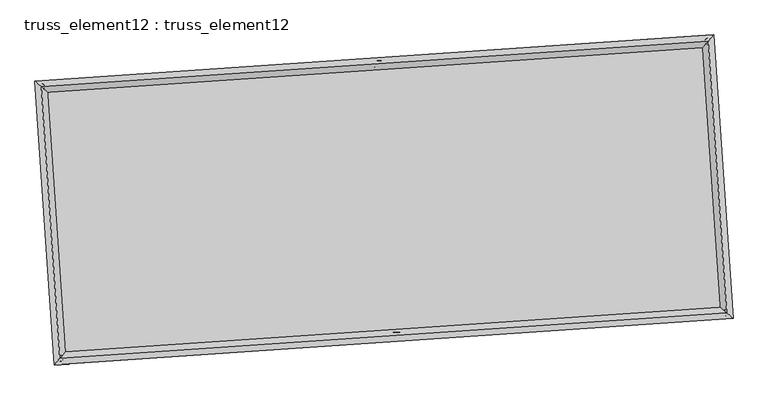
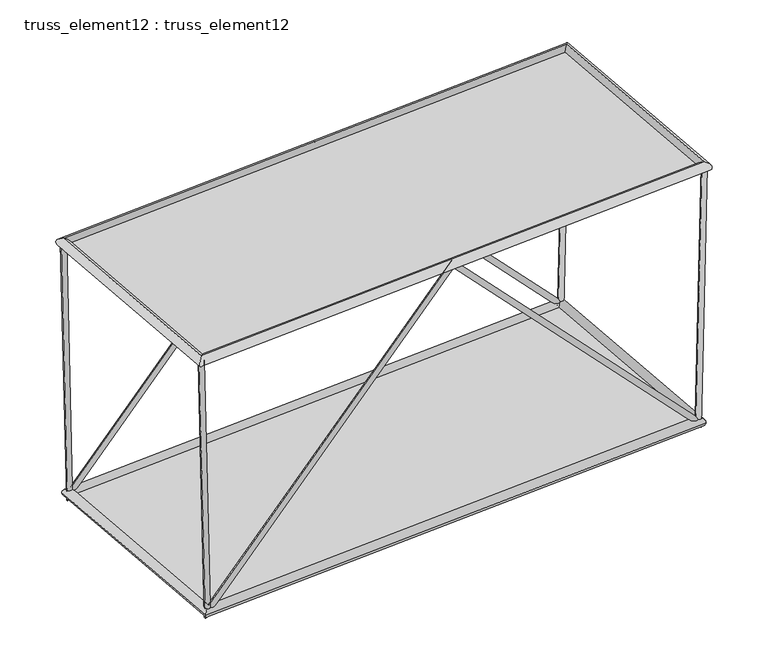
"""IFC4 building model written with IfcOpenShell, lengths in millimetres: plate geometry, truss_element12 : truss_element12."""

import ifcopenshell
import ifcopenshell.guid

model = None  # the IFC model being written
_history = None  # IfcOwnerHistory: only IFC2X3 demands one
_inside = {}  # id of a spatial element -> (the spatial element, [elements in it])
_under = {}  # id of a project, library or spatial element -> (it, [spatial elements below it])
_declared = {}  # id of a project -> (the project, [libraries it declares])
_typed = {}  # id of a type object -> (the type object, [elements of that type])
_made_of = {}  # id of a material, layer set ... -> (it, [elements and type objects made of it])


def new_model(schema):
    """Start an empty IFC model of exactly this schema.

    Asked for "IFC4X3", IfcOpenShell would pick the latest addendum, in which some entities
    have other attributes; the version numbers below select the first issue.
    IFC2X3 requires an IfcOwnerHistory on every rooted entity: one is made here for all.
    """
    global model, _history
    if schema == "IFC4X3":
        model = ifcopenshell.file(schema_version=(4, 3, 0, 0))
    else:
        model = ifcopenshell.file(schema=schema)
    _inside.clear()
    _under.clear()
    _declared.clear()
    _typed.clear()
    _made_of.clear()
    _history = None
    if model.schema == "IFC2X3":
        org = make("IfcOrganization", Name="unknown")
        user = make(
            "IfcPersonAndOrganization",
            ThePerson=make("IfcPerson", FamilyName="unknown"),
            TheOrganization=org,
        )
        app = make(
            "IfcApplication",
            ApplicationDeveloper=org,
            Version="unknown",
            ApplicationFullName="unknown",
            ApplicationIdentifier="unknown",
        )
        _history = make(
            "IfcOwnerHistory",
            OwningUser=user,
            OwningApplication=app,
            ChangeAction="ADDED",
            CreationDate=0,
        )
    return model


def make(cls, **values):
    """One entity of the class cls with the attributes given. An attribute that is None is left unset."""
    return model.create_entity(
        cls, **{name: value for name, value in values.items() if value is not None}
    )


def rooted(cls, **values):
    """An entity with a GlobalId (a new one), such as an element, a storey or a relation."""
    return make(cls, GlobalId=ifcopenshell.guid.new(), OwnerHistory=_history, **values)


def si_unit(unit_type, name, prefix=None):
    """IfcSIUnit, for example si_unit("LENGTHUNIT", "METRE", prefix="MILLI")."""
    return make("IfcSIUnit", UnitType=unit_type, Prefix=prefix, Name=name)


def assignment(units):
    """IfcUnitAssignment: the units of a project."""
    return None if units is None else make("IfcUnitAssignment", Units=units)


def point(xyz):
    """IfcCartesianPoint."""
    return None if xyz is None else make("IfcCartesianPoint", Coordinates=xyz)


def direction(xyz):
    """IfcDirection."""
    return None if xyz is None else make("IfcDirection", DirectionRatios=xyz)


def frame(location, z_axis=None, x_axis=None):
    """IfcAxis2Placement3D, a coordinate frame: its origin and axes. An axis left out is left unset."""
    return make(
        "IfcAxis2Placement3D",
        Location=point(location),
        Axis=direction(z_axis),
        RefDirection=direction(x_axis),
    )


def origin():
    """The frame at (0, 0, 0) with its axes left unset."""
    return frame((0.0, 0.0, 0.0))


def origin_with_axes():
    """The frame at (0, 0, 0) with the z axis (0, 0, 1) and the x axis (1, 0, 0) written out."""
    return frame((0.0, 0.0, 0.0), z_axis=(0.0, 0.0, 1.0), x_axis=(1.0, 0.0, 0.0))


def place(relative_to, where):
    """IfcLocalPlacement: puts the frame where relative to a parent placement (None: the world)."""
    return make(
        "IfcLocalPlacement", PlacementRelTo=relative_to, RelativePlacement=where
    )


def context(
    kind, dimensions, precision=None, world=None, true_north=None, identifier=None
):
    """IfcGeometricRepresentationContext, for example the 3D "Model" context."""
    return make(
        "IfcGeometricRepresentationContext",
        ContextIdentifier=identifier,
        ContextType=kind,
        CoordinateSpaceDimension=dimensions,
        Precision=precision,
        WorldCoordinateSystem=world,
        TrueNorth=true_north,
    )


def project(units=None, contexts=None):
    """IfcProject with its units and contexts."""
    return rooted(
        "IfcProject",
        Name="project",
        RepresentationContexts=contexts,
        UnitsInContext=assignment(units),
    )


def spatial(cls, under=None, at=None, **own):
    """A site, building, storey or space (cls), placed at a placement, below another one or the project."""
    s = rooted(cls, ObjectPlacement=at, **own)
    if under is not None:
        _under.setdefault(under.id(), (under, []))[1].append(s)
    return s


def polyline(points):
    """IfcPolyline through the points."""
    return make("IfcPolyline", Points=[point(p) for p in points])


def circle_curve(where, radius):
    """IfcCircle in the frame where."""
    return make("IfcCircle", Position=where, Radius=radius)


def ellipse_curve(where, semi_axis1, semi_axis2):
    """IfcEllipse in the frame where."""
    return make(
        "IfcEllipse", Position=where, SemiAxis1=semi_axis1, SemiAxis2=semi_axis2
    )


def outline(outer, holes=None, kind="AREA"):
    """IfcArbitraryClosedProfileDef: a profile drawn as a closed curve; with holes, ...WithVoids."""
    if holes is None:
        return make("IfcArbitraryClosedProfileDef", ProfileType=kind, OuterCurve=outer)
    return make(
        "IfcArbitraryProfileDefWithVoids",
        ProfileType=kind,
        OuterCurve=outer,
        InnerCurves=holes,
    )


def extrude(swept, where, along, depth):
    """IfcExtrudedAreaSolid: the profile swept, set in the frame where, extruded along a direction by depth."""
    return make(
        "IfcExtrudedAreaSolid",
        SweptArea=swept,
        Position=where,
        ExtrudedDirection=direction(along),
        Depth=depth,
    )


def shape(context_of_items, identifier, shape_type, items):
    """IfcShapeRepresentation: the items that make up one representation, for example the "Body"."""
    return make(
        "IfcShapeRepresentation",
        ContextOfItems=context_of_items,
        RepresentationIdentifier=identifier,
        RepresentationType=shape_type,
        Items=items,
    )


def source(mapping_origin, context_of_items, identifier, shape_type, items):
    """IfcRepresentationMap: a shape defined once, which mapped items show again and again."""
    return make(
        "IfcRepresentationMap",
        MappingOrigin=mapping_origin,
        MappedRepresentation=shape(context_of_items, identifier, shape_type, items),
    )


def transform(
    local_origin,
    x_axis=None,
    y_axis=None,
    z_axis=None,
    scale=None,
    scale2=None,
    scale3=None,
    uniform=True,
):
    """IfcCartesianTransformationOperator3D, or its non-uniform kind. x_axis, y_axis, z_axis: its Axis1, 2, 3."""
    if uniform:
        return make(
            "IfcCartesianTransformationOperator3D",
            Axis1=direction(x_axis),
            Axis2=direction(y_axis),
            LocalOrigin=point(local_origin),
            Scale=scale,
            Axis3=direction(z_axis),
        )
    return make(
        "IfcCartesianTransformationOperator3DnonUniform",
        Axis1=direction(x_axis),
        Axis2=direction(y_axis),
        LocalOrigin=point(local_origin),
        Scale=scale,
        Axis3=direction(z_axis),
        Scale2=scale2,
        Scale3=scale3,
    )


def mapped(mapping_source, mapping_target):
    """IfcMappedItem: shows the shape of a source again, moved by a transform."""
    return make(
        "IfcMappedItem", MappingSource=mapping_source, MappingTarget=mapping_target
    )


def made_of(thing, what):
    """Note that an element or type object is made of a material, layer set ...; save() writes the relation."""
    if what is not None:
        _made_of.setdefault(what.id(), (what, []))[1].append(thing)
    return thing


def element(
    cls,
    number,
    at=None,
    inside=None,
    cuts=None,
    type_object=None,
    material=None,
    context=None,
    identifier="Body",
    shape_type=None,
    held_by="IfcProductDefinitionShape",
    body=None,
    shapes=None,
    **own,
):
    """One element of the class cls, such as IfcWall. Its Tag is "e" and its number.

    at: its placement. inside: the storey or other place that contains it. cuts: it is an
    opening in that element (IfcRelVoidsElement). A single representation is given by context,
    identifier, shape_type and body (its items); several are given by shapes. held_by: the class
    of the entity that holds the representations. save() writes the other relations.
    """
    e = rooted(cls, Tag="e%d" % number, ObjectPlacement=at, **own)
    if body is not None:
        shapes = [shape(context, identifier, shape_type, body)]
    if shapes is not None:
        e.Representation = make(held_by, Representations=shapes)
    if inside is not None:
        _inside.setdefault(inside.id(), (inside, []))[1].append(e)
    if cuts is not None:
        rooted(
            "IfcRelVoidsElement", RelatingBuildingElement=cuts, RelatedOpeningElement=e
        )
    if type_object is not None:
        _typed.setdefault(type_object.id(), (type_object, []))[1].append(e)
    return made_of(e, material)


def aggregate(whole, parts):
    """IfcRelAggregates: a whole, such as a stair, and the parts it consists of."""
    return rooted("IfcRelAggregates", RelatingObject=whole, RelatedObjects=parts)


def save(model, path):
    """Write the relations noted so far, then the file.

    IfcRelAggregates (storeys below a building ...), IfcRelContainedInSpatialStructure (elements
    in a storey), IfcRelDefinesByType, IfcRelAssociatesMaterial and IfcRelDeclares: one each for
    every whole, place, type object, material and project.
    """
    for whole, parts in _under.values():
        aggregate(whole, parts)
    for where, things in _inside.values():
        rooted(
            "IfcRelContainedInSpatialStructure",
            RelatedElements=things,
            RelatingStructure=where,
        )
    for kind, things in _typed.values():
        rooted("IfcRelDefinesByType", RelatedObjects=things, RelatingType=kind)
    for what, things in _made_of.values():
        rooted("IfcRelAssociatesMaterial", RelatedObjects=things, RelatingMaterial=what)
    for by, libraries in _declared.values():
        rooted("IfcRelDeclares", RelatingContext=by, RelatedDefinitions=libraries)
    model.write(path)


def plane_surface(at):
    """IfcPlane: the flat surface through the origin of the frame at, square to its z axis."""
    return make("IfcPlane", Position=at)


def cylinder_surface(at, radius):
    """IfcCylindricalSurface: all points at the distance radius from the z axis of the frame at."""
    return make("IfcCylindricalSurface", Position=at, Radius=radius)


def advanced_brep(points, edges, surfaces, faces):
    """IfcAdvancedBrep: a solid bounded by faces that lie on surfaces and meet in shared edges.

    An edge is (start, end): straight between two places in points (the first is 0);
    or (start, end, curve); or (start, end, curve, False) where it runs against its curve.
    A face is (place in surfaces, loops), or (place, loops, False) where it looks against
    its surface's normal. A loop lists edges by number (the first is 1), with a minus sign
    where the edge is run from its end to its start. The first loop is the outer one.
    """
    corners = [point(p) for p in points]
    vertices = [make("IfcVertexPoint", VertexGeometry=c) for c in corners]
    made = []
    for start, end, *more in edges:
        made.append(
            make(
                "IfcEdgeCurve",
                EdgeStart=vertices[start],
                EdgeEnd=vertices[end],
                EdgeGeometry=more[0] if more else make("IfcPolyline", Points=[corners[start], corners[end]]),
                SameSense=more[1] if len(more) > 1 else True,
            )
        )
    hull = []
    for where, loops, *sense in faces:
        bounds = []
        for j, loop in enumerate(loops):
            ring = [make("IfcOrientedEdge", EdgeElement=made[abs(k) - 1], Orientation=k > 0) for k in loop]
            bounds.append(
                make(
                    "IfcFaceOuterBound" if j == 0 else "IfcFaceBound",
                    Bound=make("IfcEdgeLoop", EdgeList=ring),
                    Orientation=True,
                )
            )
        hull.append(make("IfcAdvancedFace", Bounds=bounds, FaceSurface=surfaces[where], SameSense=sense[0] if sense else True))
    return make("IfcAdvancedBrep", Outer=make("IfcClosedShell", CfsFaces=hull))


def truss_element12_truss_element12_a9ba9ad0(model_context):
    return source(origin(), model_context, "Body", "SolidModel", [
        advanced_brep(
        [(-3781.0066057, 2268.3099305, 4999.8074441), (-3880.0830312, 2254.9505451, 4997.4860818), (-3667.7432726, 2276.0329266, 121.2492765), (-3761.2436102, 2263.0537535, -121.2492765), (1063.9114307, 2598.6664741, 5070.7560558), (1064.3567641, 2592.0930992, 4926.5285654), (5795.1912206, 2921.2744577, 121.2466741), (5889.5697565, 2921.1060308, -121.2466741), (5908.826689, 2929.0228283, 4999.8023514), (6008.7993375, 2929.2358427, 4997.4733651)],
        [
            (0, 1, circle_curve(frame((-3830.5448184, 2261.6302378, 4998.6467629), z_axis=(-0.023210275405575107, -0.0015826204493892785, 0.9997293525890447), x_axis=(-0.1335944347975753, 0.9910349023519434, -0.0015327463556159752)), 50.0)),
            (1, 0, circle_curve(frame((-3830.5448184, 2261.6302378, 4998.6467629), z_axis=(-0.023210275405575107, -0.0015826204493892785, 0.9997293525890447), x_axis=(-0.1335944347975753, 0.9910349023519434, -0.0015327463556159752)), 50.0)),
            (0, 2),
            (2, 3, ellipse_curve(frame((-3714.4934414, 2269.54334, 0.0), z_axis=(-0.9300246539008389, -0.06341484579481178, 0.3619843925771457), x_axis=(0.36114581811246804, 0.024625160493310073, 0.9321841553741164)), 130.3533132, 50.0)),
            (3, 1),
            (3, 2, ellipse_curve(frame((-3714.4934414, 2269.54334, 0.0), z_axis=(-0.9300246539008389, -0.06341484579481178, 0.3619843925771457), x_axis=(0.36114581811246804, 0.024625160493310073, 0.9321841553741164)), 130.3533132, 50.0)),
            (2, 4),
            (4, 5, ellipse_curve(frame((1064.1340974, 2595.3797867, 4998.6423106), z_axis=(-0.9976833958768766, -0.06802823821520107, 1.99228329783538e-05), x_axis=(-1.9876679665461313e-05, -1.3553152281554114e-06, -0.9999999998015403)), 72.2707708, 50.0)),
            (5, 3),
            (5, 4, ellipse_curve(frame((1064.1340974, 2595.3797867, 4998.6423106), z_axis=(-0.9976833958768766, -0.06802823821520107, 1.99228329783538e-05), x_axis=(-1.9876679665461313e-05, -1.3553152281554114e-06, -0.9999999998015403)), 72.2707708, 50.0)),
            (4, 6),
            (6, 7, ellipse_curve(frame((5842.3804885, 2921.1902443, 0.0), z_axis=(-0.930045648078386, -0.06341627730797217, -0.36193019805323456), x_axis=(-0.3610917491358036, -0.02462147373532669, 0.9322051982997877)), 130.347573, 50.0)),
            (7, 5),
            (7, 6, ellipse_curve(frame((5842.3804885, 2921.1902443, 0.0), z_axis=(-0.930045648078386, -0.06341627730797217, -0.36193019805323456), x_axis=(-0.3610917491358036, -0.02462147373532669, 0.9322051982997877)), 130.347573, 50.0)),
            (8, 9, circle_curve(frame((5958.8130133, 2929.1293355, 4998.6378583), z_axis=(0.023286504957413055, 0.001587818252753427, 0.9997275716514297), x_axis=(-0.002166543517392095, 0.9999964706541518, -0.0015377803573986969)), 50.0)),
            (9, 8, circle_curve(frame((5958.8130133, 2929.1293355, 4998.6378583), z_axis=(0.023286504957413055, 0.001587818252753427, 0.9997275716514297), x_axis=(-0.002166543517392095, 0.9999964706541518, -0.0015377803573986969)), 50.0)),
            (6, 8),
            (9, 7),
        ],
        [
            plane_surface(frame((-3830.5448184, 2311.6301752, 4998.7259153), z_axis=(-0.023210275405573556, -0.0015826204493892511, 0.9997293525890448), x_axis=(0.9997306052710387, -3.674295485112113e-05, 0.023210246322644693))),
            cylinder_surface(frame((-3830.5448184, 2261.6302378, 4998.6467629), z_axis=(-0.02321027540557511, -0.001582620449389279, 0.9997293525890449), x_axis=(-0.1335944347975753, 0.9910349023519434, -0.0015327463556159752)), 50.0),
            cylinder_surface(frame((-3714.4934414, 2269.54334, 0.0), z_axis=(-0.6902542548350474, -0.04706581373513176, -0.7220345371653379), x_axis=(-0.02041980494214943, 0.9987518501447402, -0.04558259973480142)), 50.0),
            cylinder_surface(frame((1064.1340974, 2595.3797867, 4998.6423106), z_axis=(-0.6902255509886974, -0.04706385652896254, 0.7220621040956036), x_axis=(-0.11534286833238303, 0.9922794072885053, -0.04558070420727685)), 50.0),
            plane_surface(frame((5958.8130133, 2879.1293986, 4998.7172707), z_axis=(0.023286504957412656, 0.0015878182527521501, 0.99972757165143), x_axis=(0.9997288325775489, -3.698476667857163e-05, -0.023286475586886003))),
            cylinder_surface(frame((5842.3804885, 2921.1902443, 0.0), z_axis=(-0.023286504957413058, -0.0015878182527534275, -0.9997275716514299), x_axis=(-0.002166543517392095, 0.9999964706541518, -0.0015377803573986969)), 50.0),
        ],
        [
            (0, [[1, 2]]),
            (1, [[-1, 3, 4, 5]]),
            (1, [[-2, -5, 6, -3]]),
            (2, [[-4, 7, 8, 9]]),
            (2, [[-6, -9, 10, -7]]),
            (3, [[-8, 11, 12, 13]]),
            (3, [[-10, -13, 14, -11]]),
            (4, [[15, 16]]),
            (5, [[-12, 17, -16, 18]]),
            (5, [[-14, -18, -15, -17]]),
        ],
    ),
        advanced_brep(
        [(-3508.8936528, -1722.4236538, 4999.8074441), (-3607.9700783, -1735.7830392, 4997.4860818), (-3395.6303197, -1714.7006577, 121.2492765), (-3489.1306573, -1727.6798308, -121.2492765), (1336.0243837, -1392.0671102, 5070.7560558), (1336.469717, -1398.6404851, 4926.5285654), (6067.3041735, -1069.4591266, 121.2466741), (6161.6827094, -1069.6275535, -121.2466741), (6180.939642, -1061.710756, 4999.8023514), (6280.9122905, -1061.4977416, 4997.4733651)],
        [
            (0, 1, circle_curve(frame((-3558.4318655, -1729.1033465, 4998.6467629), z_axis=(-0.023210275405574413, -0.001582620449389233, 0.9997293525890448), x_axis=(-0.13359443479757582, 0.9910349023519432, -0.0015327463556159403)), 50.0)),
            (1, 0, circle_curve(frame((-3558.4318655, -1729.1033465, 4998.6467629), z_axis=(-0.023210275405574413, -0.001582620449389233, 0.9997293525890448), x_axis=(-0.13359443479757582, 0.9910349023519432, -0.0015327463556159403)), 50.0)),
            (0, 2),
            (2, 3, ellipse_curve(frame((-3442.3804885, -1721.1902443, 0.0), z_axis=(-0.9300246539008385, -0.06341484579481202, 0.36198439257714643), x_axis=(0.3611458181124687, 0.024625160493310223, 0.9321841553741161)), 130.3533132, 50.0)),
            (3, 1),
            (3, 2, ellipse_curve(frame((-3442.3804885, -1721.1902443, 0.0), z_axis=(-0.9300246539008385, -0.06341484579481202, 0.36198439257714643), x_axis=(0.3611458181124687, 0.024625160493310223, 0.9321841553741161)), 130.3533132, 50.0)),
            (2, 4),
            (4, 5, ellipse_curve(frame((1336.2470503, -1395.3537976, 4998.6423106), z_axis=(-0.9976833958768766, -0.06802823821520144, 1.9922832978915455e-05), x_axis=(-1.9876679665922593e-05, -1.3553152280977514e-06, -0.9999999998015403)), 72.2707708, 50.0)),
            (5, 3),
            (5, 4, ellipse_curve(frame((1336.2470503, -1395.3537976, 4998.6423106), z_axis=(-0.9976833958768766, -0.06802823821520144, 1.9922832978915455e-05), x_axis=(-1.9876679665922593e-05, -1.3553152280977514e-06, -0.9999999998015403)), 72.2707708, 50.0)),
            (4, 6),
            (6, 7, ellipse_curve(frame((6114.4934414, -1069.54334, 0.0), z_axis=(-0.930045648078386, -0.0634162773079726, -0.36193019805323406), x_axis=(-0.3610917491358033, -0.02462147373532683, 0.9322051982997878)), 130.347573, 50.0)),
            (7, 5),
            (7, 6, ellipse_curve(frame((6114.4934414, -1069.54334, 0.0), z_axis=(-0.930045648078386, -0.0634162773079726, -0.36193019805323406), x_axis=(-0.3610917491358033, -0.02462147373532683, 0.9322051982997878)), 130.347573, 50.0)),
            (8, 9, circle_curve(frame((6230.9259662, -1061.6042488, 4998.6378583), z_axis=(0.023286504957413627, 0.0015878182527534774, 0.9997275716514298), x_axis=(-0.0021665435173920953, 0.9999964706541518, -0.0015377803573987457)), 50.0)),
            (9, 8, circle_curve(frame((6230.9259662, -1061.6042488, 4998.6378583), z_axis=(0.023286504957413627, 0.0015878182527534774, 0.9997275716514298), x_axis=(-0.0021665435173920953, 0.9999964706541518, -0.0015377803573987457)), 50.0)),
            (6, 8),
            (9, 7),
        ],
        [
            plane_surface(frame((-3558.4318655, -1679.1034091, 4998.7259153), z_axis=(-0.023210275405573556, -0.0015826204493892427, 0.9997293525890448), x_axis=(0.9997306052710387, -3.674295485112113e-05, 0.023210246322644693))),
            cylinder_surface(frame((-3558.4318655, -1729.1033465, 4998.6467629), z_axis=(-0.023210275405574413, -0.001582620449389233, 0.9997293525890448), x_axis=(-0.13359443479757582, 0.9910349023519432, -0.0015327463556159403)), 50.0),
            cylinder_surface(frame((-3442.3804885, -1721.1902443, 0.0), z_axis=(-0.6902542548350478, -0.04706581373513197, -0.7220345371653374), x_axis=(-0.020419804942149452, 0.9987518501447401, -0.0455825997348017)), 50.0),
            cylinder_surface(frame((1336.2470503, -1395.3537976, 4998.6423106), z_axis=(-0.6902255509886973, -0.04706385652896285, 0.7220621040956039), x_axis=(-0.11534286833238368, 0.9922794072885052, -0.04558070420727702)), 50.0),
            plane_surface(frame((6230.9259662, -1111.6041857, 4998.7172707), z_axis=(0.023286504957412656, 0.001587818252752135, 0.99972757165143), x_axis=(0.9997288325775489, -3.698476667812754e-05, -0.023286475586886003))),
            cylinder_surface(frame((6114.4934414, -1069.54334, 0.0), z_axis=(-0.023286504957413627, -0.0015878182527534774, -0.9997275716514298), x_axis=(-0.0021665435173920953, 0.9999964706541518, -0.0015377803573987457)), 50.0),
        ],
        [
            (0, [[1, 2]]),
            (1, [[-1, 3, 4, 5]]),
            (1, [[-2, -5, 6, -3]]),
            (2, [[-4, 7, 8, 9]]),
            (2, [[-6, -9, 10, -7]]),
            (3, [[-8, 11, 12, 13]]),
            (3, [[-10, -13, 14, -11]]),
            (4, [[15, 16]]),
            (5, [[-12, 17, -16, 18]]),
            (5, [[-14, -18, -15, -17]]),
        ],
    ),
        advanced_brep(
        [(-3558.4341768, -1729.1059081, 4908.646763), (-3558.4295543, -1729.1007848, 5088.6467629), (-3830.5421809, 2261.6280136, 5088.6467629), (-3830.547456, 2261.632462, 4908.646763), (5958.810865, 2929.126785, 5088.6378582), (5958.8151616, 2929.1318861, 4908.6378583), (6230.9234916, -1061.6020135, 5088.6378582), (6230.9284408, -1061.6064841, 4908.6378583)],
        [
            (0, 1, ellipse_curve(frame((-3558.4318655, -1729.1033465, 4998.6467629), z_axis=(-0.7535719234051691, 0.6573654662780984, 6.417150933687899e-07), x_axis=(-0.657365466277788, -0.7535719234054401, 6.417150933687674e-07)), 127.2792206, 90.0)),
            (1, 2),
            (2, 3, ellipse_curve(frame((-3830.5448184, 2261.6302378, 4998.6467629), z_axis=(-0.6573654662777882, -0.7535719234054399, 6.417150933687475e-07), x_axis=(0.753571923405169, -0.6573654662780987, -6.417150933687697e-07)), 127.2792206, 90.0)),
            (3, 0),
            (1, 0, ellipse_curve(frame((-3558.4318655, -1729.1033465, 4998.6467629), z_axis=(-0.7535719234051691, 0.6573654662780984, 6.417150933687899e-07), x_axis=(-0.657365466277788, -0.7535719234054401, 6.417150933687674e-07)), 127.2792206, 90.0)),
            (3, 2, ellipse_curve(frame((-3830.5448184, 2261.6302378, 4998.6467629), z_axis=(-0.6573654662777882, -0.7535719234054399, 6.417150933687475e-07), x_axis=(0.753571923405169, -0.6573654662780987, -6.417150933687697e-07)), 127.2792206, 90.0)),
            (2, 4),
            (4, 5, ellipse_curve(frame((5958.8130133, 2929.1293355, 4998.6378583), z_axis=(-0.7535719234051688, 0.6573654662780991, 6.417150933687491e-07), x_axis=(-0.6573654662777887, -0.7535719234054395, 6.417150933687683e-07)), 127.2792206, 90.0)),
            (5, 3),
            (5, 4, ellipse_curve(frame((5958.8130133, 2929.1293355, 4998.6378583), z_axis=(-0.7535719234051688, 0.6573654662780991, 6.417150933687491e-07), x_axis=(-0.6573654662777887, -0.7535719234054395, 6.417150933687683e-07)), 127.2792206, 90.0)),
            (4, 6),
            (6, 7, ellipse_curve(frame((6230.9259662, -1061.6042488, 4998.6378583), z_axis=(0.6573654662777887, 0.7535719234054394, -6.417150933687883e-07), x_axis=(-0.7535719234051687, 0.6573654662780992, 6.41715093368769e-07)), 127.2792206, 90.0)),
            (7, 5),
            (7, 6, ellipse_curve(frame((6230.9259662, -1061.6042488, 4998.6378583), z_axis=(0.6573654662777887, 0.7535719234054394, -6.417150933687883e-07), x_axis=(-0.7535719234051687, 0.6573654662780992, 6.41715093368769e-07)), 127.2792206, 90.0)),
            (6, 1),
            (0, 7),
        ],
        [
            cylinder_surface(frame((-3558.4318655, -1729.1033465, 4998.6467629), z_axis=(0.0680282382287046, -0.9976833960748763, 0.0), x_axis=(-0.9976833956960517, -0.068028238202874, 2.7557367220821674e-05)), 90.0),
            cylinder_surface(frame((-3830.5448184, 2261.6302378, 4998.6467629), z_axis=(-0.9976833960744657, -0.06802823822867518, 9.075221882216156e-07), x_axis=(-0.06802823818041658, 0.9976833957222373, 2.6649845032922314e-05)), 90.0),
            cylinder_surface(frame((5958.8130133, 2929.1293355, 4998.6378583), z_axis=(-0.06802823822870338, 0.9976833960748765, 0.0), x_axis=(0.9976833957443104, 0.06802823820616334, 2.5742322845022958e-05)), 90.0),
            cylinder_surface(frame((6230.9259662, -1061.6042488, 4998.6378583), z_axis=(0.9976833960744657, 0.06802823822867522, -9.07522188221644e-07), x_axis=(0.06802823822867522, -0.9976833957189467, 2.6649845032922317e-05)), 90.0),
        ],
        [
            (0, [[1, 2, 3, 4]]),
            (0, [[5, -4, 6, -2]]),
            (1, [[-3, 7, 8, 9]]),
            (1, [[-6, -9, 10, -7]]),
            (2, [[-8, 11, 12, 13]]),
            (2, [[-10, -13, 14, -11]]),
            (3, [[-12, 15, -1, 16]]),
            (3, [[-14, -16, -5, -15]]),
        ],
    ),
        advanced_brep(
        [(-3358.7115243, -1625.2761972, 0.0), (-3526.0494527, -1817.1042913, 0.0), (-3810.4074885, 2353.2123043, 0.0), (-3618.5793943, 2185.8743758, 0.0), (5926.0494527, 3017.1042913, 0.0), (5758.7115243, 2825.2761972, 0.0), (6210.4074885, -1153.2123043, 0.0), (6018.5793943, -985.8743758, 0.0)],
        [
            (0, 1, ellipse_curve(frame((-3442.3804885, -1721.1902443, 0.0), z_axis=(-0.7535719234054589, 0.6573654662780797, 0.0), x_axis=(-0.6573654662780796, -0.753571923405459, 0.0)), 127.2792206, 90.0)),
            (1, 2),
            (2, 3, ellipse_curve(frame((-3714.4934414, 2269.54334, 0.0), z_axis=(-0.6573654662780798, -0.7535719234054586, 0.0), x_axis=(0.7535719234054585, -0.6573654662780801, 0.0)), 127.2792206, 90.0)),
            (3, 0),
            (1, 0, ellipse_curve(frame((-3442.3804885, -1721.1902443, 0.0), z_axis=(-0.7535719234054589, 0.6573654662780797, 0.0), x_axis=(-0.6573654662780796, -0.753571923405459, 0.0)), 127.2792206, 90.0)),
            (3, 2, ellipse_curve(frame((-3714.4934414, 2269.54334, 0.0), z_axis=(-0.6573654662780798, -0.7535719234054586, 0.0), x_axis=(0.7535719234054585, -0.6573654662780801, 0.0)), 127.2792206, 90.0)),
            (2, 4),
            (4, 5, ellipse_curve(frame((5842.3804885, 2921.1902443, 0.0), z_axis=(-0.7535719234054585, 0.6573654662780802, 0.0), x_axis=(-0.6573654662780801, -0.7535719234054584, 0.0)), 127.2792206, 90.0)),
            (5, 3),
            (5, 4, ellipse_curve(frame((5842.3804885, 2921.1902443, 0.0), z_axis=(-0.7535719234054585, 0.6573654662780802, 0.0), x_axis=(-0.6573654662780801, -0.7535719234054584, 0.0)), 127.2792206, 90.0)),
            (4, 6),
            (6, 7, ellipse_curve(frame((6114.4934414, -1069.54334, 0.0), z_axis=(0.65736546627808, 0.7535719234054586, 0.0), x_axis=(-0.7535719234054588, 0.6573654662780799, 0.0)), 127.2792206, 90.0)),
            (7, 5),
            (7, 6, ellipse_curve(frame((6114.4934414, -1069.54334, 0.0), z_axis=(0.65736546627808, 0.7535719234054586, 0.0), x_axis=(-0.7535719234054588, 0.6573654662780799, 0.0)), 127.2792206, 90.0)),
            (6, 1),
            (0, 7),
        ],
        [
            cylinder_surface(frame((-3442.3804885, -1721.1902443, 0.0), z_axis=(0.068028238228703, -0.9976833960748764, 0.0), x_axis=(-0.9976833960748764, -0.068028238228703, 0.0)), 90.0),
            cylinder_surface(frame((-3714.4934414, 2269.54334, 0.0), z_axis=(-0.9976833960748765, -0.06802823822870191, 0.0), x_axis=(-0.06802823822870191, 0.9976833960748765, 0.0)), 90.0),
            cylinder_surface(frame((5842.3804885, 2921.1902443, 0.0), z_axis=(-0.06802823822870221, 0.9976833960748765, 0.0), x_axis=(0.9976833960748765, 0.06802823822870221, 0.0)), 90.0),
            cylinder_surface(frame((6114.4934414, -1069.54334, 0.0), z_axis=(0.9976833960748765, 0.0680282382287023, 0.0), x_axis=(0.0680282382287023, -0.9976833960748765, 0.0)), 90.0),
        ],
        [
            (0, [[1, 2, 3, 4]]),
            (0, [[5, -4, 6, -2]]),
            (1, [[-3, 7, 8, 9]]),
            (1, [[-6, -9, 10, -7]]),
            (2, [[-8, 11, 12, 13]]),
            (2, [[-10, -13, 14, -11]]),
            (3, [[-12, 15, -1, 16]]),
            (3, [[-14, -16, -5, -15]]),
        ],
    ),
        extrude(outline(polyline([(-3442.3804885, -1721.1902443), (-3714.4934414, 2269.54334), (5842.3804885, 2921.1902443), (6114.4934414, -1069.54334), (-3442.3804885, -1721.1902443)])), origin_with_axes(), (0.0, 0.0, 1.0), 20.0),
        extrude(outline(polyline([(-2000.0, 4906.0442773), (2000.0, 4906.0442773), (2000.0, -4906.0442773), (-2000.0, -4906.0442773), (-2000.0, 4906.0442773)])), frame((1200.1905739, 600.0129945, 4998.6423106), z_axis=(9.054198187582591e-07, 6.173713561817491e-08, 0.9999999999995882), x_axis=(-0.068028238228703, 0.9976833960748764, 0.0)), (0.0, 0.0, 1.0), 20.0),
    ])


if __name__ == "__main__":
    model = new_model("IFC4")
    model_context = context("Model", 3, world=origin())
    ifc_project = project(units=[si_unit("LENGTHUNIT", "METRE", prefix="MILLI")], contexts=[model_context])
    site = spatial("IfcSite", under=ifc_project)
    building = spatial("IfcBuilding", under=site)
    placement = place(None, origin())
    truss_element12_truss_element12_shape = truss_element12_truss_element12_a9ba9ad0(model_context)
    element("IfcPlate", 1, ObjectType="truss_element12 : truss_element12", at=placement, inside=building, context=model_context, shape_type="MappedRepresentation", body=[
        mapped(truss_element12_truss_element12_shape, transform((0.0, 0.0, 0.0), x_axis=(1.0, 0.0, 0.0), y_axis=(0.0, 1.0, 0.0), z_axis=(0.0, 0.0, 1.0))),
    ])
    save(model, "model.ifc")

# Revit data of these elements
# Type "truss_element12 : truss_element12"
#   steellbar1 = 90 mm
#   steelbar2 = 50 mm
#   offset1 = 5000 mm
#   M = Default Roof
# Element 1 (IfcPlate, "truss_element12 : truss_element12")
#   Materials on its faces: "Default Roof"
# Materials
#   "Default Roof": class "Miscellaneous", colour RGB 0 127 0, transparency 0, Comments = "Rendering appearance not upgraded Rendering appearance not upgraded ", Cost = 0
